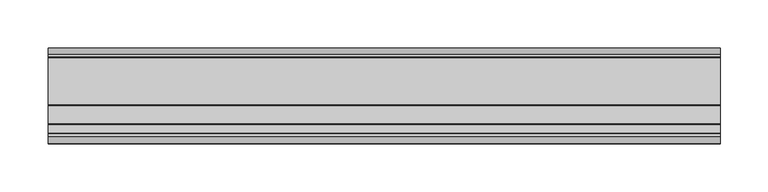
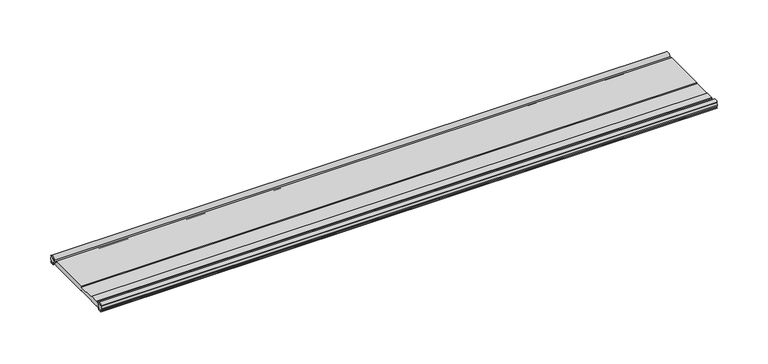
"""IFC4 building model written with IfcOpenShell, lengths in millimetres: proxy geometry, TN_Гидрошпонка ТН Фундамент : Гидрошпонка ТН Фундамент ТПС-В 100-2."""

from ifc_helpers import new_model, si_unit, point, frame, frame_2d, origin, place, context, project, spatial, polyline, circle_curve, trimmed, segment, composite_curve, outline, extrude, source, transform, mapped, element, save


def specialty_equipment_d68811da(model_context):
    return source(origin(), model_context, "Body", "SweptSolid", [
        extrude(outline(composite_curve([segment(trimmed(circle_curve(frame_2d((-47.0, 1.9826107)), 3.0), [point((-50.0, 1.9826107))], [point((-44.0, 1.9826107))], False, "CARTESIAN"), True, "CONTINUOUS"), segment(trimmed(circle_curve(frame_2d((-47.0, 1.9826107)), 3.0), [point((-44.0, 1.9826107))], [point((-50.0, 1.9826107))], False, "CARTESIAN"), True, "CONTINUOUS")], self_intersect=False)), frame((0.0, 0.0, 0.0), z_axis=(1.0, 0.0, 0.0), x_axis=(0.0, 1.0, 0.0)), (0.0, 0.0, 1.0), 700.0),
        extrude(outline(composite_curve([segment(polyline([(-42.9110191, 4.0), (-40.0400595, 4.0), (-39.3329528, 4.7071068), (-30.3626141, 4.7071068), (-29.6555073, 4.0), (-10.4400654, 4.0), (-9.7329586, 4.7071068), (39.4275825, 4.7071068), (40.1346893, 4.0), (42.9110191, 4.0)]), True, "CONTINUOUS"), segment(trimmed(circle_curve(frame_2d((46.7376194, 2.9019073)), 3.9810398), [point((42.9110191, 4.0))], [point((49.8730463, 5.3550229))], False, "CARTESIAN"), True, "CONTINUOUS"), segment(polyline([(49.8730463, 5.3550229), (49.1845402, 4.6665169)]), True, "CONTINUOUS"), segment(trimmed(circle_curve(frame_2d((47.0, 1.9826107)), 3.4605734), [point((49.1845402, 4.6665169))], [point((49.1845402, -0.7012955))], True, "CARTESIAN"), True, "CONTINUOUS"), segment(polyline([(49.1845402, -0.7012955), (49.8907254, -1.4074807)]), True, "CONTINUOUS"), segment(trimmed(circle_curve(frame_2d((46.7376194, 1.0142478)), 3.9757825), [point((49.8907254, -1.4074807))], [point((42.8933837, 0.0))], False, "CARTESIAN"), True, "CONTINUOUS"), segment(polyline([(42.8933837, 0.0), (40.1346893, 0.0), (39.39555, -0.7391394), (-9.7329586, -0.7391394), (-10.472098, 0.0), (-29.6555073, 0.0), (-30.3946467, -0.7391394), (-39.3329528, -0.7391394), (-40.0720921, 0.0), (-42.8933837, 0.0)]), True, "CONTINUOUS"), segment(trimmed(circle_curve(frame_2d((-46.7376194, 1.0142478)), 3.9757825), [point((-42.8933837, 0.0))], [point((-49.8907254, -1.4074807))], False, "CARTESIAN"), True, "CONTINUOUS"), segment(polyline([(-49.8907254, -1.4074807), (-49.1845402, -0.7012955)]), True, "CONTINUOUS"), segment(trimmed(circle_curve(frame_2d((-47.0, 1.9826107)), 3.4605734), [point((-49.1845402, -0.7012955))], [point((-49.1845402, 4.6665169))], True, "CARTESIAN"), True, "CONTINUOUS"), segment(polyline([(-49.1845402, 4.6665169), (-49.8730463, 5.3550229)]), True, "CONTINUOUS"), segment(trimmed(circle_curve(frame_2d((-46.7376194, 2.9019073)), 3.9810398), [point((-49.8730463, 5.3550229))], [point((-42.9110191, 4.0))], False, "CARTESIAN"), True, "CONTINUOUS")], self_intersect=False)), frame((0.0, 0.0, 0.0), z_axis=(1.0, 0.0, 0.0), x_axis=(0.0, 1.0, 0.0)), (0.0, 0.0, 1.0), 700.0),
        extrude(outline(composite_curve([segment(trimmed(circle_curve(frame_2d((47.0, 1.9826107)), 3.0), [point((44.0, 1.9826107))], [point((50.0, 1.9826107))], False, "CARTESIAN"), True, "CONTINUOUS"), segment(trimmed(circle_curve(frame_2d((47.0, 1.9826107)), 3.0), [point((50.0, 1.9826107))], [point((44.0, 1.9826107))], False, "CARTESIAN"), True, "CONTINUOUS")], self_intersect=False)), frame((0.0, 0.0, 0.0), z_axis=(1.0, 0.0, 0.0), x_axis=(0.0, 1.0, 0.0)), (0.0, 0.0, 1.0), 700.0),
    ])


if __name__ == "__main__":
    model = new_model("IFC4")
    model_context = context("Model", 3, world=origin())
    ifc_project = project(units=[si_unit("LENGTHUNIT", "METRE", prefix="MILLI")], contexts=[model_context])
    site = spatial("IfcSite", under=ifc_project)
    building = spatial("IfcBuilding", under=site)
    placement = place(None, origin())
    specialty_equipment_shape = specialty_equipment_d68811da(model_context)
    element("IfcBuildingElementProxy", 1, Name="TN_Гидрошпонка ТН Фундамент : Гидрошпонка ТН Фундамент ТПС-В 100-2", ObjectType="TN_Гидрошпонка ТН Фундамент : Гидрошпонка ТН Фундамент ТПС-В 100-2", at=placement, inside=building, context=model_context, shape_type="MappedRepresentation", body=[
        mapped(specialty_equipment_shape, transform((0.0, 0.0, 0.0), x_axis=(1.0, 0.0, 0.0), y_axis=(0.0, 1.0, 0.0), z_axis=(0.0, 0.0, 1.0))),
    ])
    save(model, "model.ifc")

# Revit data of these elements
# Type "TN_Гидрошпонка ТН Фундамент : Гидрошпонка ТН Фундамент ТПС-В 100-2"
#   Description = "Внутренние гидроизоляционные шпонки ТН Фундамент ТПС-В предназначены для герметизации технологических швов бетонирования в местах сопряжения плиты и стены фундамента при строительстве подземных и заглубленных конструкций зданий и сооружений различного назначения и класса ответственности. Наличие набухающего шнура на краях шпонки позволяет повысить надежность шва."
#   Type Comments = "п.м."
#   Manufacturer = "ТехноНИКОЛЬ"
#   URL = "https://nav.tn.ru/catalog/gidroizolyatsiya/komplektatsiya-dlya-gidroizolyatsii/gidroshponki-tekhnonikol-fundament-tps-v/"
#   ADSK_Примечание = ""
#   ADSK_Обозначение [instance default] = "ТехноНИКОЛЬ"
#   ADSK_Наименование = "Гидрошпонка ТН Фундамент ТПС-В 100-2"
#   ADSK_Масса_Текст = ""
#   ADSK_Марка = ""
#   ADSK_Код изделия = "66666"
#   ADSK_Завод-изготовитель [instance default] = "ТехноНИКОЛЬ"
#   ADSK_Единица измерения [instance default] = "п.м."
#   ADSK_Группирование = "Гидрошпонки"
#   ADSK_URL страницы изделия = "https://nav.tn.ru/catalog/gidroizolyatsiya/komplektatsiya-dlya-gidroizolyatsii/gidroshponki-tekhnonikol-fundament-tps-v/"
#   ADSK_URL документации изделия = "https://nav.tn.ru/upload/iblock/39e/n34lwlimw5x5s3mf7b0hwzc10sm1ot3v/Tekhlist-7.400_Gidroshponki-TN-Fundament-TPS_V_RU_ru.pdf"
#   built-in parameter 1001306 [instance default] = 3.28084 (stored number, unit not read)
#   ADSK_Размер_Длина [instance default] = 1000 mm
#   ADSK_Количество [instance default] = 1
#   Гидрошпонка ТН Фундамент ТШ-Н-210 = no
#   Гидрошпонка ТН Фундамент ДШП-В-50 = no
#   Гидрошпонка ТН Фундамент ДШП-В-20 = no
#   Гидрошпонка ТН Фундамент ДШ-В-280 = no
#   Гидрошпонка ТН Фундамент ДШ-В-250 = no
#   Гидрошпонка ТН Фундамент ТШ-В-250 = no
#   Гидрошпонка ТН Фундамент ТПС-В 140-1 = no
#   Гидрошпонка ТН Фундамент ДШ-Н-280 = no
#   Гидрошпонка ТН Фундамент ДШ-Н-250 = no
#   Гидрошпонка ТН Фундамент ТПС-В 100-2 = yes
#   Гидрошпонка ТН Фундамент ТШ-Н-250 = no
#   Гидрошпонка ТН Фундамент ТШ-В-210 = no
#   Материал = TN_ПВХ_Черный
#   Default Elevation = 0
# Element 1 (IfcBuildingElementProxy, "TN_Гидрошпонка ТН Фундамент : Гидрошпонка ТН Фундамент ТПС-В 100-2")
#   built-in parameter 1001306 = 2.29659 (stored number, unit not read)
#   ADSK_Размер_Длина = 700 mm
#   ADSK_Количество = 0.7
#   Materials on its faces: "TN_ПВХ_Черный"
# Materials
#   "TN_ПВХ_Черный": class "Типовые", colour RGB 48 48 48, transparency 0, Cost = 0
